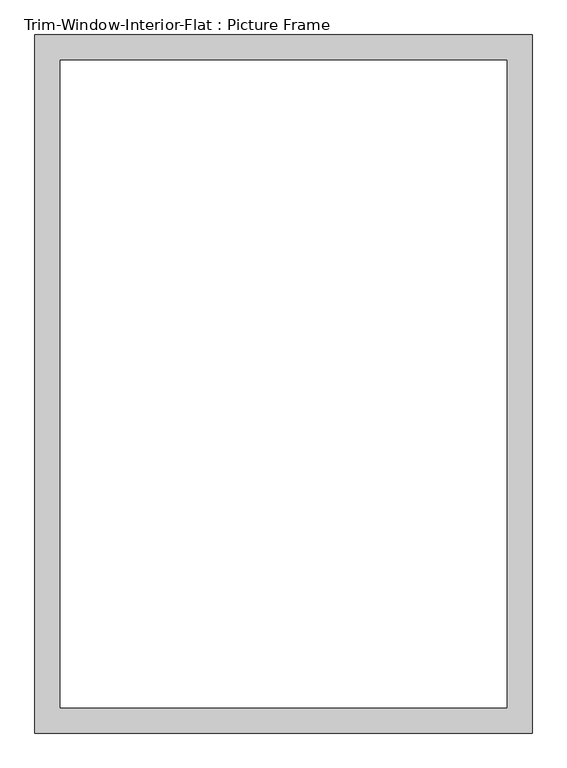
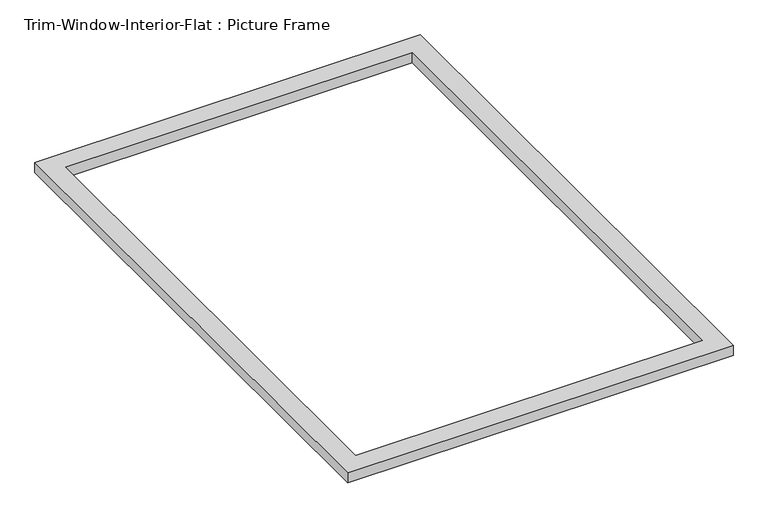
"""IFC4 building model written with IfcOpenShell, lengths in millimetres: proxy geometry, Trim-Window-Interior-Flat : Picture Frame."""

from ifc_helpers import new_model, si_unit, origin, origin_with_axes, place, context, project, spatial, polyline, outline, extrude, source, transform, mapped, element, save


def trim_window_interior_flat_picture_frame_208726ef(model_context):
    return source(origin(), model_context, "Body", "SweptSolid", [
        extrude(outline(polyline([(565.15, 44.45), (565.15, -1543.05), (-565.15, -1543.05), (-565.15, 44.45), (565.15, 44.45)]), holes=[polyline([(508.0, -12.7), (-508.0, -12.7), (-508.0, -1485.9), (508.0, -1485.9), (508.0, -12.7)])]), origin_with_axes(), (0.0, 0.0, 1.0), 31.75),
    ])


if __name__ == "__main__":
    model = new_model("IFC4")
    model_context = context("Model", 3, world=origin())
    ifc_project = project(units=[si_unit("LENGTHUNIT", "METRE", prefix="MILLI")], contexts=[model_context])
    site = spatial("IfcSite", under=ifc_project)
    building = spatial("IfcBuilding", under=site)
    placement = place(None, origin())
    trim_window_interior_flat_picture_frame_shape = trim_window_interior_flat_picture_frame_208726ef(model_context)
    element("IfcBuildingElementProxy", 1, Name="Trim-Window-Interior-Flat : Picture Frame", ObjectType="Trim-Window-Interior-Flat : Picture Frame", at=placement, inside=building, context=model_context, shape_type="MappedRepresentation", body=[
        mapped(trim_window_interior_flat_picture_frame_shape, transform((0.0, 0.0, 0.0), x_axis=(1.0, 0.0, 0.0), y_axis=(0.0, 1.0, 0.0), z_axis=(0.0, 0.0, 1.0))),
    ])
    save(model, "model.ifc")

# Revit data of these elements
# Type "Trim-Window-Interior-Flat : Picture Frame"
#   Trim Thickness_Picture Frame = 0' - 1 1/4"
#   Trim Width = 0' - 2 1/4"
#   Trim Thickness_with Sill = 0' - 0 3/4"
#   Sill Thickness = 0' - 1 1/4"
#   Opening Width [instance default] = 2' - 0"
#   Opening Height [instance default] = 3' - 0"
#   Default Elevation = 4' - 0"
#   Sill = no
#   Picture Frame = yes
#   Trim Material [instance default] = none
# Element 1 (IfcBuildingElementProxy, "Trim-Window-Interior-Flat : Picture Frame")
#   Opening Width = 3' - 5"
#   Opening Height = 4' - 11"
#   Trim Material = 1X WOOD COMPOSITE TRIM
#   Materials on its faces: "1X WOOD COMPOSITE TRIM"
# Materials
#   "1X WOOD COMPOSITE TRIM": class "Generic", colour RGB 88 61 61, transparency 0, Cost = 0
